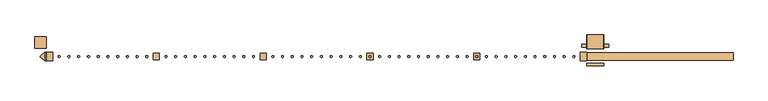
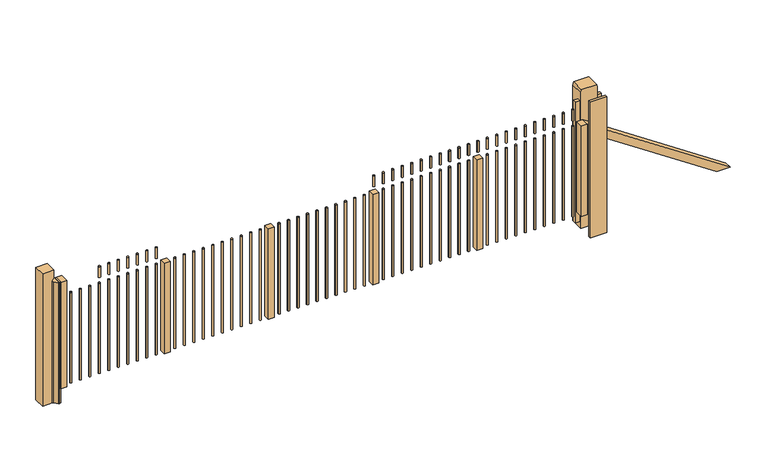
"""IFC4 building model written with IfcOpenShell, lengths in millimetres: door geometry, NLRS_90_DO_UN_schuifpoort met spijlen_gen_rsf : schuifpoort automatisch bxh 7000x1800-NP."""

import ifcopenshell
import ifcopenshell.guid

model = None  # the IFC model being written
_history = None  # IfcOwnerHistory: only IFC2X3 demands one
_inside = {}  # id of a spatial element -> (the spatial element, [elements in it])
_under = {}  # id of a project, library or spatial element -> (it, [spatial elements below it])
_declared = {}  # id of a project -> (the project, [libraries it declares])
_typed = {}  # id of a type object -> (the type object, [elements of that type])
_made_of = {}  # id of a material, layer set ... -> (it, [elements and type objects made of it])


def new_model(schema):
    """Start an empty IFC model of exactly this schema.

    Asked for "IFC4X3", IfcOpenShell would pick the latest addendum, in which some entities
    have other attributes; the version numbers below select the first issue.
    IFC2X3 requires an IfcOwnerHistory on every rooted entity: one is made here for all.
    """
    global model, _history
    if schema == "IFC4X3":
        model = ifcopenshell.file(schema_version=(4, 3, 0, 0))
    else:
        model = ifcopenshell.file(schema=schema)
    _inside.clear()
    _under.clear()
    _declared.clear()
    _typed.clear()
    _made_of.clear()
    _history = None
    if model.schema == "IFC2X3":
        org = make("IfcOrganization", Name="unknown")
        user = make(
            "IfcPersonAndOrganization",
            ThePerson=make("IfcPerson", FamilyName="unknown"),
            TheOrganization=org,
        )
        app = make(
            "IfcApplication",
            ApplicationDeveloper=org,
            Version="unknown",
            ApplicationFullName="unknown",
            ApplicationIdentifier="unknown",
        )
        _history = make(
            "IfcOwnerHistory",
            OwningUser=user,
            OwningApplication=app,
            ChangeAction="ADDED",
            CreationDate=0,
        )
    return model


def make(cls, **values):
    """One entity of the class cls with the attributes given. An attribute that is None is left unset."""
    return model.create_entity(
        cls, **{name: value for name, value in values.items() if value is not None}
    )


def rooted(cls, **values):
    """An entity with a GlobalId (a new one), such as an element, a storey or a relation."""
    return make(cls, GlobalId=ifcopenshell.guid.new(), OwnerHistory=_history, **values)


def si_unit(unit_type, name, prefix=None):
    """IfcSIUnit, for example si_unit("LENGTHUNIT", "METRE", prefix="MILLI")."""
    return make("IfcSIUnit", UnitType=unit_type, Prefix=prefix, Name=name)


def assignment(units):
    """IfcUnitAssignment: the units of a project."""
    return None if units is None else make("IfcUnitAssignment", Units=units)


def point(xyz):
    """IfcCartesianPoint."""
    return None if xyz is None else make("IfcCartesianPoint", Coordinates=xyz)


def direction(xyz):
    """IfcDirection."""
    return None if xyz is None else make("IfcDirection", DirectionRatios=xyz)


def frame(location, z_axis=None, x_axis=None):
    """IfcAxis2Placement3D, a coordinate frame: its origin and axes. An axis left out is left unset."""
    return make(
        "IfcAxis2Placement3D",
        Location=point(location),
        Axis=direction(z_axis),
        RefDirection=direction(x_axis),
    )


def frame_2d(location, x_axis=None):
    """IfcAxis2Placement2D, a coordinate frame in the plane: its origin and x axis."""
    return make(
        "IfcAxis2Placement2D", Location=point(location), RefDirection=direction(x_axis)
    )


def origin():
    """The frame at (0, 0, 0) with its axes left unset."""
    return frame((0.0, 0.0, 0.0))


def place(relative_to, where):
    """IfcLocalPlacement: puts the frame where relative to a parent placement (None: the world)."""
    return make(
        "IfcLocalPlacement", PlacementRelTo=relative_to, RelativePlacement=where
    )


def context(
    kind, dimensions, precision=None, world=None, true_north=None, identifier=None
):
    """IfcGeometricRepresentationContext, for example the 3D "Model" context."""
    return make(
        "IfcGeometricRepresentationContext",
        ContextIdentifier=identifier,
        ContextType=kind,
        CoordinateSpaceDimension=dimensions,
        Precision=precision,
        WorldCoordinateSystem=world,
        TrueNorth=true_north,
    )


def project(units=None, contexts=None):
    """IfcProject with its units and contexts."""
    return rooted(
        "IfcProject",
        Name="project",
        RepresentationContexts=contexts,
        UnitsInContext=assignment(units),
    )


def spatial(cls, under=None, at=None, **own):
    """A site, building, storey or space (cls), placed at a placement, below another one or the project."""
    s = rooted(cls, ObjectPlacement=at, **own)
    if under is not None:
        _under.setdefault(under.id(), (under, []))[1].append(s)
    return s


def polyline(points):
    """IfcPolyline through the points."""
    return make("IfcPolyline", Points=[point(p) for p in points])


def circle_curve(where, radius):
    """IfcCircle in the frame where."""
    return make("IfcCircle", Position=where, Radius=radius)


def trimmed(basis, trim1, trim2, sense, master):
    """IfcTrimmedCurve: the piece of a basis curve between two trims."""
    return make(
        "IfcTrimmedCurve",
        BasisCurve=basis,
        Trim1=trim1,
        Trim2=trim2,
        SenseAgreement=sense,
        MasterRepresentation=master,
    )


def segment(curve, same_sense, transition):
    """IfcCompositeCurveSegment."""
    return make(
        "IfcCompositeCurveSegment",
        Transition=transition,
        SameSense=same_sense,
        ParentCurve=curve,
    )


def composite_curve(segments, self_intersect=None):
    """IfcCompositeCurve: segments joined end to end."""
    return make("IfcCompositeCurve", Segments=segments, SelfIntersect=self_intersect)


def outline(outer, holes=None, kind="AREA"):
    """IfcArbitraryClosedProfileDef: a profile drawn as a closed curve; with holes, ...WithVoids."""
    if holes is None:
        return make("IfcArbitraryClosedProfileDef", ProfileType=kind, OuterCurve=outer)
    return make(
        "IfcArbitraryProfileDefWithVoids",
        ProfileType=kind,
        OuterCurve=outer,
        InnerCurves=holes,
    )


def extrude(swept, where, along, depth):
    """IfcExtrudedAreaSolid: the profile swept, set in the frame where, extruded along a direction by depth."""
    return make(
        "IfcExtrudedAreaSolid",
        SweptArea=swept,
        Position=where,
        ExtrudedDirection=direction(along),
        Depth=depth,
    )


def shape(context_of_items, identifier, shape_type, items):
    """IfcShapeRepresentation: the items that make up one representation, for example the "Body"."""
    return make(
        "IfcShapeRepresentation",
        ContextOfItems=context_of_items,
        RepresentationIdentifier=identifier,
        RepresentationType=shape_type,
        Items=items,
    )


def source(mapping_origin, context_of_items, identifier, shape_type, items):
    """IfcRepresentationMap: a shape defined once, which mapped items show again and again."""
    return make(
        "IfcRepresentationMap",
        MappingOrigin=mapping_origin,
        MappedRepresentation=shape(context_of_items, identifier, shape_type, items),
    )


def transform(
    local_origin,
    x_axis=None,
    y_axis=None,
    z_axis=None,
    scale=None,
    scale2=None,
    scale3=None,
    uniform=True,
):
    """IfcCartesianTransformationOperator3D, or its non-uniform kind. x_axis, y_axis, z_axis: its Axis1, 2, 3."""
    if uniform:
        return make(
            "IfcCartesianTransformationOperator3D",
            Axis1=direction(x_axis),
            Axis2=direction(y_axis),
            LocalOrigin=point(local_origin),
            Scale=scale,
            Axis3=direction(z_axis),
        )
    return make(
        "IfcCartesianTransformationOperator3DnonUniform",
        Axis1=direction(x_axis),
        Axis2=direction(y_axis),
        LocalOrigin=point(local_origin),
        Scale=scale,
        Axis3=direction(z_axis),
        Scale2=scale2,
        Scale3=scale3,
    )


def mapped(mapping_source, mapping_target):
    """IfcMappedItem: shows the shape of a source again, moved by a transform."""
    return make(
        "IfcMappedItem", MappingSource=mapping_source, MappingTarget=mapping_target
    )


def made_of(thing, what):
    """Note that an element or type object is made of a material, layer set ...; save() writes the relation."""
    if what is not None:
        _made_of.setdefault(what.id(), (what, []))[1].append(thing)
    return thing


def element(
    cls,
    number,
    at=None,
    inside=None,
    cuts=None,
    type_object=None,
    material=None,
    context=None,
    identifier="Body",
    shape_type=None,
    held_by="IfcProductDefinitionShape",
    body=None,
    shapes=None,
    **own,
):
    """One element of the class cls, such as IfcWall. Its Tag is "e" and its number.

    at: its placement. inside: the storey or other place that contains it. cuts: it is an
    opening in that element (IfcRelVoidsElement). A single representation is given by context,
    identifier, shape_type and body (its items); several are given by shapes. held_by: the class
    of the entity that holds the representations. save() writes the other relations.
    """
    e = rooted(cls, Tag="e%d" % number, ObjectPlacement=at, **own)
    if body is not None:
        shapes = [shape(context, identifier, shape_type, body)]
    if shapes is not None:
        e.Representation = make(held_by, Representations=shapes)
    if inside is not None:
        _inside.setdefault(inside.id(), (inside, []))[1].append(e)
    if cuts is not None:
        rooted(
            "IfcRelVoidsElement", RelatingBuildingElement=cuts, RelatedOpeningElement=e
        )
    if type_object is not None:
        _typed.setdefault(type_object.id(), (type_object, []))[1].append(e)
    return made_of(e, material)


def aggregate(whole, parts):
    """IfcRelAggregates: a whole, such as a stair, and the parts it consists of."""
    return rooted("IfcRelAggregates", RelatingObject=whole, RelatedObjects=parts)


def save(model, path):
    """Write the relations noted so far, then the file.

    IfcRelAggregates (storeys below a building ...), IfcRelContainedInSpatialStructure (elements
    in a storey), IfcRelDefinesByType, IfcRelAssociatesMaterial and IfcRelDeclares: one each for
    every whole, place, type object, material and project.
    """
    for whole, parts in _under.values():
        aggregate(whole, parts)
    for where, things in _inside.values():
        rooted(
            "IfcRelContainedInSpatialStructure",
            RelatedElements=things,
            RelatingStructure=where,
        )
    for kind, things in _typed.values():
        rooted("IfcRelDefinesByType", RelatedObjects=things, RelatingType=kind)
    for what, things in _made_of.values():
        rooted("IfcRelAssociatesMaterial", RelatedObjects=things, RelatingMaterial=what)
    for by, libraries in _declared.values():
        rooted("IfcRelDeclares", RelatingContext=by, RelatedDefinitions=libraries)
    model.write(path)


def door_7189267d(model_context):
    return source(origin(), model_context, "Body", "SweptSolid", [
        extrude(outline(composite_curve([segment(trimmed(circle_curve(frame_2d((3299.5, 0.0)), 12.5), [point((3312.0, 0.0))], [point((3287.0, 0.0))], False, "CARTESIAN"), True, "CONTINUOUS"), segment(trimmed(circle_curve(frame_2d((3299.5, 0.0)), 12.5), [point((3287.0, 0.0))], [point((3312.0, 0.0))], False, "CARTESIAN"), True, "CONTINUOUS")], self_intersect=False)), frame((0.0, 0.0, 300.0), z_axis=(0.0, 0.0, 1.0), x_axis=(1.0, 0.0, 0.0)), (0.0, 0.0, 1.0), 1270.0),
        extrude(outline(composite_curve([segment(trimmed(circle_curve(frame_2d((3173.5, 0.0)), 12.5), [point((3186.0, 0.0))], [point((3161.0, 0.0))], False, "CARTESIAN"), True, "CONTINUOUS"), segment(trimmed(circle_curve(frame_2d((3173.5, 0.0)), 12.5), [point((3161.0, 0.0))], [point((3186.0, 0.0))], False, "CARTESIAN"), True, "CONTINUOUS")], self_intersect=False)), frame((0.0, 0.0, 300.0), z_axis=(0.0, 0.0, 1.0), x_axis=(1.0, 0.0, 0.0)), (0.0, 0.0, 1.0), 1270.0),
        extrude(outline(composite_curve([segment(trimmed(circle_curve(frame_2d((3047.5, 0.0)), 12.5), [point((3060.0, 0.0))], [point((3035.0, 0.0))], False, "CARTESIAN"), True, "CONTINUOUS"), segment(trimmed(circle_curve(frame_2d((3047.5, 0.0)), 12.5), [point((3035.0, 0.0))], [point((3060.0, 0.0))], False, "CARTESIAN"), True, "CONTINUOUS")], self_intersect=False)), frame((0.0, 0.0, 300.0), z_axis=(0.0, 0.0, 1.0), x_axis=(1.0, 0.0, 0.0)), (0.0, 0.0, 1.0), 1270.0),
        extrude(outline(composite_curve([segment(trimmed(circle_curve(frame_2d((2921.5, 0.0)), 12.5), [point((2934.0, 0.0))], [point((2909.0, 0.0))], False, "CARTESIAN"), True, "CONTINUOUS"), segment(trimmed(circle_curve(frame_2d((2921.5, 0.0)), 12.5), [point((2909.0, 0.0))], [point((2934.0, 0.0))], False, "CARTESIAN"), True, "CONTINUOUS")], self_intersect=False)), frame((0.0, 0.0, 300.0), z_axis=(0.0, 0.0, 1.0), x_axis=(1.0, 0.0, 0.0)), (0.0, 0.0, 1.0), 1270.0),
        extrude(outline(composite_curve([segment(trimmed(circle_curve(frame_2d((2795.5, 0.0)), 12.5), [point((2808.0, 0.0))], [point((2783.0, 0.0))], False, "CARTESIAN"), True, "CONTINUOUS"), segment(trimmed(circle_curve(frame_2d((2795.5, 0.0)), 12.5), [point((2783.0, 0.0))], [point((2808.0, 0.0))], False, "CARTESIAN"), True, "CONTINUOUS")], self_intersect=False)), frame((0.0, 0.0, 300.0), z_axis=(0.0, 0.0, 1.0), x_axis=(1.0, 0.0, 0.0)), (0.0, 0.0, 1.0), 1270.0),
        extrude(outline(composite_curve([segment(trimmed(circle_curve(frame_2d((2669.5, 0.0)), 12.5), [point((2682.0, 0.0))], [point((2657.0, 0.0))], False, "CARTESIAN"), True, "CONTINUOUS"), segment(trimmed(circle_curve(frame_2d((2669.5, 0.0)), 12.5), [point((2657.0, 0.0))], [point((2682.0, 0.0))], False, "CARTESIAN"), True, "CONTINUOUS")], self_intersect=False)), frame((0.0, 0.0, 300.0), z_axis=(0.0, 0.0, 1.0), x_axis=(1.0, 0.0, 0.0)), (0.0, 0.0, 1.0), 1270.0),
        extrude(outline(composite_curve([segment(trimmed(circle_curve(frame_2d((2543.5, 0.0)), 12.5), [point((2556.0, 0.0))], [point((2531.0, 0.0))], False, "CARTESIAN"), True, "CONTINUOUS"), segment(trimmed(circle_curve(frame_2d((2543.5, 0.0)), 12.5), [point((2531.0, 0.0))], [point((2556.0, 0.0))], False, "CARTESIAN"), True, "CONTINUOUS")], self_intersect=False)), frame((0.0, 0.0, 300.0), z_axis=(0.0, 0.0, 1.0), x_axis=(1.0, 0.0, 0.0)), (0.0, 0.0, 1.0), 1270.0),
        extrude(outline(composite_curve([segment(trimmed(circle_curve(frame_2d((2417.5, 0.0)), 12.5), [point((2430.0, 0.0))], [point((2405.0, 0.0))], False, "CARTESIAN"), True, "CONTINUOUS"), segment(trimmed(circle_curve(frame_2d((2417.5, 0.0)), 12.5), [point((2405.0, 0.0))], [point((2430.0, 0.0))], False, "CARTESIAN"), True, "CONTINUOUS")], self_intersect=False)), frame((0.0, 0.0, 300.0), z_axis=(0.0, 0.0, 1.0), x_axis=(1.0, 0.0, 0.0)), (0.0, 0.0, 1.0), 1270.0),
        extrude(outline(composite_curve([segment(trimmed(circle_curve(frame_2d((2291.5, 0.0)), 12.5), [point((2304.0, 0.0))], [point((2279.0, 0.0))], False, "CARTESIAN"), True, "CONTINUOUS"), segment(trimmed(circle_curve(frame_2d((2291.5, 0.0)), 12.5), [point((2279.0, 0.0))], [point((2304.0, 0.0))], False, "CARTESIAN"), True, "CONTINUOUS")], self_intersect=False)), frame((0.0, 0.0, 300.0), z_axis=(0.0, 0.0, 1.0), x_axis=(1.0, 0.0, 0.0)), (0.0, 0.0, 1.0), 1270.0),
        extrude(outline(composite_curve([segment(trimmed(circle_curve(frame_2d((2165.5, 0.0)), 12.5), [point((2178.0, 0.0))], [point((2153.0, 0.0))], False, "CARTESIAN"), True, "CONTINUOUS"), segment(trimmed(circle_curve(frame_2d((2165.5, 0.0)), 12.5), [point((2153.0, 0.0))], [point((2178.0, 0.0))], False, "CARTESIAN"), True, "CONTINUOUS")], self_intersect=False)), frame((0.0, 0.0, 300.0), z_axis=(0.0, 0.0, 1.0), x_axis=(1.0, 0.0, 0.0)), (0.0, 0.0, 1.0), 1270.0),
        extrude(outline(composite_curve([segment(trimmed(circle_curve(frame_2d((1915.5, 0.0)), 12.5), [point((1928.0, 0.0))], [point((1903.0, 0.0))], False, "CARTESIAN"), True, "CONTINUOUS"), segment(trimmed(circle_curve(frame_2d((1915.5, 0.0)), 12.5), [point((1903.0, 0.0))], [point((1928.0, 0.0))], False, "CARTESIAN"), True, "CONTINUOUS")], self_intersect=False)), frame((0.0, 0.0, 300.0), z_axis=(0.0, 0.0, 1.0), x_axis=(1.0, 0.0, 0.0)), (0.0, 0.0, 1.0), 1270.0),
        extrude(outline(composite_curve([segment(trimmed(circle_curve(frame_2d((1789.5, 0.0)), 12.5), [point((1802.0, 0.0))], [point((1777.0, 0.0))], False, "CARTESIAN"), True, "CONTINUOUS"), segment(trimmed(circle_curve(frame_2d((1789.5, 0.0)), 12.5), [point((1777.0, 0.0))], [point((1802.0, 0.0))], False, "CARTESIAN"), True, "CONTINUOUS")], self_intersect=False)), frame((0.0, 0.0, 300.0), z_axis=(0.0, 0.0, 1.0), x_axis=(1.0, 0.0, 0.0)), (0.0, 0.0, 1.0), 1270.0),
        extrude(outline(composite_curve([segment(trimmed(circle_curve(frame_2d((1663.5, 0.0)), 12.5), [point((1676.0, 0.0))], [point((1651.0, 0.0))], False, "CARTESIAN"), True, "CONTINUOUS"), segment(trimmed(circle_curve(frame_2d((1663.5, 0.0)), 12.5), [point((1651.0, 0.0))], [point((1676.0, 0.0))], False, "CARTESIAN"), True, "CONTINUOUS")], self_intersect=False)), frame((0.0, 0.0, 300.0), z_axis=(0.0, 0.0, 1.0), x_axis=(1.0, 0.0, 0.0)), (0.0, 0.0, 1.0), 1270.0),
        extrude(outline(composite_curve([segment(trimmed(circle_curve(frame_2d((1537.5, 0.0)), 12.5), [point((1550.0, 0.0))], [point((1525.0, 0.0))], False, "CARTESIAN"), True, "CONTINUOUS"), segment(trimmed(circle_curve(frame_2d((1537.5, 0.0)), 12.5), [point((1525.0, 0.0))], [point((1550.0, 0.0))], False, "CARTESIAN"), True, "CONTINUOUS")], self_intersect=False)), frame((0.0, 0.0, 300.0), z_axis=(0.0, 0.0, 1.0), x_axis=(1.0, 0.0, 0.0)), (0.0, 0.0, 1.0), 1270.0),
        extrude(outline(composite_curve([segment(trimmed(circle_curve(frame_2d((1411.5, 0.0)), 12.5), [point((1424.0, 0.0))], [point((1399.0, 0.0))], False, "CARTESIAN"), True, "CONTINUOUS"), segment(trimmed(circle_curve(frame_2d((1411.5, 0.0)), 12.5), [point((1399.0, 0.0))], [point((1424.0, 0.0))], False, "CARTESIAN"), True, "CONTINUOUS")], self_intersect=False)), frame((0.0, 0.0, 300.0), z_axis=(0.0, 0.0, 1.0), x_axis=(1.0, 0.0, 0.0)), (0.0, 0.0, 1.0), 1270.0),
        extrude(outline(composite_curve([segment(trimmed(circle_curve(frame_2d((1285.5, 0.0)), 12.5), [point((1298.0, 0.0))], [point((1273.0, 0.0))], False, "CARTESIAN"), True, "CONTINUOUS"), segment(trimmed(circle_curve(frame_2d((1285.5, 0.0)), 12.5), [point((1273.0, 0.0))], [point((1298.0, 0.0))], False, "CARTESIAN"), True, "CONTINUOUS")], self_intersect=False)), frame((0.0, 0.0, 300.0), z_axis=(0.0, 0.0, 1.0), x_axis=(1.0, 0.0, 0.0)), (0.0, 0.0, 1.0), 1270.0),
        extrude(outline(composite_curve([segment(trimmed(circle_curve(frame_2d((1159.5, 0.0)), 12.5), [point((1172.0, 0.0))], [point((1147.0, 0.0))], False, "CARTESIAN"), True, "CONTINUOUS"), segment(trimmed(circle_curve(frame_2d((1159.5, 0.0)), 12.5), [point((1147.0, 0.0))], [point((1172.0, 0.0))], False, "CARTESIAN"), True, "CONTINUOUS")], self_intersect=False)), frame((0.0, 0.0, 300.0), z_axis=(0.0, 0.0, 1.0), x_axis=(1.0, 0.0, 0.0)), (0.0, 0.0, 1.0), 1270.0),
        extrude(outline(composite_curve([segment(trimmed(circle_curve(frame_2d((1033.5, 0.0)), 12.5), [point((1046.0, 0.0))], [point((1021.0, 0.0))], False, "CARTESIAN"), True, "CONTINUOUS"), segment(trimmed(circle_curve(frame_2d((1033.5, 0.0)), 12.5), [point((1021.0, 0.0))], [point((1046.0, 0.0))], False, "CARTESIAN"), True, "CONTINUOUS")], self_intersect=False)), frame((0.0, 0.0, 300.0), z_axis=(0.0, 0.0, 1.0), x_axis=(1.0, 0.0, 0.0)), (0.0, 0.0, 1.0), 1270.0),
        extrude(outline(composite_curve([segment(trimmed(circle_curve(frame_2d((907.5, 0.0)), 12.5), [point((920.0, 0.0))], [point((895.0, 0.0))], False, "CARTESIAN"), True, "CONTINUOUS"), segment(trimmed(circle_curve(frame_2d((907.5, 0.0)), 12.5), [point((895.0, 0.0))], [point((920.0, 0.0))], False, "CARTESIAN"), True, "CONTINUOUS")], self_intersect=False)), frame((0.0, 0.0, 300.0), z_axis=(0.0, 0.0, 1.0), x_axis=(1.0, 0.0, 0.0)), (0.0, 0.0, 1.0), 1270.0),
        extrude(outline(composite_curve([segment(trimmed(circle_curve(frame_2d((781.5, 0.0)), 12.5), [point((794.0, 0.0))], [point((769.0, 0.0))], False, "CARTESIAN"), True, "CONTINUOUS"), segment(trimmed(circle_curve(frame_2d((781.5, 0.0)), 12.5), [point((769.0, 0.0))], [point((794.0, 0.0))], False, "CARTESIAN"), True, "CONTINUOUS")], self_intersect=False)), frame((0.0, 0.0, 300.0), z_axis=(0.0, 0.0, 1.0), x_axis=(1.0, 0.0, 0.0)), (0.0, 0.0, 1.0), 1270.0),
        extrude(outline(polyline([(3465.0, 158.5), (3465.0, 118.5), (3400.0, 118.5), (3400.0, 158.5), (3465.0, 158.5)])), frame((0.0, 0.0, 100.0), z_axis=(0.0, 0.0, 1.0), x_axis=(1.0, 0.0, 0.0)), (0.0, 0.0, 1.0), 1700.0),
        extrude(outline(polyline([(3685.0, 158.5), (3750.0, 158.5), (3750.0, 118.5), (3685.0, 118.5), (3685.0, 158.5)])), frame((0.0, 0.0, 100.0), z_axis=(0.0, 0.0, 1.0), x_axis=(1.0, 0.0, 0.0)), (0.0, 0.0, 1.0), 1700.0),
        extrude(outline(polyline([(3685.0, -84.5), (3685.0, -119.5), (3465.0, -119.5), (3465.0, -84.5), (3685.0, -84.5)])), frame((0.0, 0.0, 12.0), z_axis=(0.0, 0.0, 1.0), x_axis=(1.0, 0.0, 0.0)), (0.0, 0.0, 1.0), 1906.0),
        extrude(outline(polyline([(1918.0, 3465.0), (12.0, 3465.0), (12.0, 3685.0), (1918.0, 3685.0), (1960.0, 3677.5), (1960.0, 3472.5), (1918.0, 3465.0)])), frame((0.0, 100.5, 0.0), z_axis=(0.0, 1.0, 0.0), x_axis=(0.0, 0.0, 1.0)), (0.0, 0.0, 1.0), 180.0),
        extrude(outline(polyline([(2000.5, 40.0), (2080.5, 40.0), (2080.5, -40.0), (2000.5, -40.0), (2000.5, 40.0)])), frame((0.0, 0.0, 300.0), z_axis=(0.0, 0.0, 1.0), x_axis=(1.0, 0.0, 0.0)), (0.0, 0.0, 1.0), 1270.0),
        extrude(outline(polyline([(616.5, 40.0), (696.5, 40.0), (696.5, -40.0), (616.5, -40.0), (616.5, 40.0)])), frame((0.0, 0.0, 300.0), z_axis=(0.0, 0.0, 1.0), x_axis=(1.0, 0.0, 0.0)), (0.0, 0.0, 1.0), 1270.0),
        extrude(outline(polyline([(-767.5, 40.0), (-687.5, 40.0), (-687.5, -40.0), (-767.5, -40.0), (-767.5, 40.0)])), frame((0.0, 0.0, 300.0), z_axis=(0.0, 0.0, 1.0), x_axis=(1.0, 0.0, 0.0)), (0.0, 0.0, 1.0), 1270.0),
        extrude(outline(polyline([(-2151.5, 40.0), (-2071.5, 40.0), (-2071.5, -40.0), (-2151.5, -40.0), (-2151.5, 40.0)])), frame((0.0, 0.0, 300.0), z_axis=(0.0, 0.0, 1.0), x_axis=(1.0, 0.0, 0.0)), (0.0, 0.0, 1.0), 1270.0),
        extrude(outline(composite_curve([segment(trimmed(circle_curve(frame_2d((531.5, 0.0)), 12.5), [point((544.0, 0.0))], [point((519.0, 0.0))], False, "CARTESIAN"), True, "CONTINUOUS"), segment(trimmed(circle_curve(frame_2d((531.5, 0.0)), 12.5), [point((519.0, 0.0))], [point((544.0, 0.0))], False, "CARTESIAN"), True, "CONTINUOUS")], self_intersect=False)), frame((0.0, 0.0, 300.0), z_axis=(0.0, 0.0, 1.0), x_axis=(1.0, 0.0, 0.0)), (0.0, 0.0, 1.0), 1270.0),
        extrude(outline(composite_curve([segment(trimmed(circle_curve(frame_2d((405.5, 0.0)), 12.5), [point((418.0, 0.0))], [point((393.0, 0.0))], False, "CARTESIAN"), True, "CONTINUOUS"), segment(trimmed(circle_curve(frame_2d((405.5, 0.0)), 12.5), [point((393.0, 0.0))], [point((418.0, 0.0))], False, "CARTESIAN"), True, "CONTINUOUS")], self_intersect=False)), frame((0.0, 0.0, 300.0), z_axis=(0.0, 0.0, 1.0), x_axis=(1.0, 0.0, 0.0)), (0.0, 0.0, 1.0), 1270.0),
        extrude(outline(composite_curve([segment(trimmed(circle_curve(frame_2d((279.5, 0.0)), 12.5), [point((292.0, 0.0))], [point((267.0, 0.0))], False, "CARTESIAN"), True, "CONTINUOUS"), segment(trimmed(circle_curve(frame_2d((279.5, 0.0)), 12.5), [point((267.0, 0.0))], [point((292.0, 0.0))], False, "CARTESIAN"), True, "CONTINUOUS")], self_intersect=False)), frame((0.0, 0.0, 300.0), z_axis=(0.0, 0.0, 1.0), x_axis=(1.0, 0.0, 0.0)), (0.0, 0.0, 1.0), 1270.0),
        extrude(outline(composite_curve([segment(trimmed(circle_curve(frame_2d((153.5, 0.0)), 12.5), [point((166.0, 0.0))], [point((141.0, 0.0))], False, "CARTESIAN"), True, "CONTINUOUS"), segment(trimmed(circle_curve(frame_2d((153.5, 0.0)), 12.5), [point((141.0, 0.0))], [point((166.0, 0.0))], False, "CARTESIAN"), True, "CONTINUOUS")], self_intersect=False)), frame((0.0, 0.0, 300.0), z_axis=(0.0, 0.0, 1.0), x_axis=(1.0, 0.0, 0.0)), (0.0, 0.0, 1.0), 1270.0),
        extrude(outline(composite_curve([segment(trimmed(circle_curve(frame_2d((27.5, 0.0)), 12.5), [point((40.0, 0.0))], [point((15.0, 0.0))], False, "CARTESIAN"), True, "CONTINUOUS"), segment(trimmed(circle_curve(frame_2d((27.5, 0.0)), 12.5), [point((15.0, 0.0))], [point((40.0, 0.0))], False, "CARTESIAN"), True, "CONTINUOUS")], self_intersect=False)), frame((0.0, 0.0, 300.0), z_axis=(0.0, 0.0, 1.0), x_axis=(1.0, 0.0, 0.0)), (0.0, 0.0, 1.0), 1270.0),
        extrude(outline(composite_curve([segment(trimmed(circle_curve(frame_2d((-98.5, 0.0)), 12.5), [point((-86.0, 0.0))], [point((-111.0, 0.0))], False, "CARTESIAN"), True, "CONTINUOUS"), segment(trimmed(circle_curve(frame_2d((-98.5, 0.0)), 12.5), [point((-111.0, 0.0))], [point((-86.0, 0.0))], False, "CARTESIAN"), True, "CONTINUOUS")], self_intersect=False)), frame((0.0, 0.0, 300.0), z_axis=(0.0, 0.0, 1.0), x_axis=(1.0, 0.0, 0.0)), (0.0, 0.0, 1.0), 1270.0),
        extrude(outline(composite_curve([segment(trimmed(circle_curve(frame_2d((-224.5, 0.0)), 12.5), [point((-212.0, 0.0))], [point((-237.0, 0.0))], False, "CARTESIAN"), True, "CONTINUOUS"), segment(trimmed(circle_curve(frame_2d((-224.5, 0.0)), 12.5), [point((-237.0, 0.0))], [point((-212.0, 0.0))], False, "CARTESIAN"), True, "CONTINUOUS")], self_intersect=False)), frame((0.0, 0.0, 300.0), z_axis=(0.0, 0.0, 1.0), x_axis=(1.0, 0.0, 0.0)), (0.0, 0.0, 1.0), 1270.0),
        extrude(outline(composite_curve([segment(trimmed(circle_curve(frame_2d((-350.5, 0.0)), 12.5), [point((-338.0, 0.0))], [point((-363.0, 0.0))], False, "CARTESIAN"), True, "CONTINUOUS"), segment(trimmed(circle_curve(frame_2d((-350.5, 0.0)), 12.5), [point((-363.0, 0.0))], [point((-338.0, 0.0))], False, "CARTESIAN"), True, "CONTINUOUS")], self_intersect=False)), frame((0.0, 0.0, 300.0), z_axis=(0.0, 0.0, 1.0), x_axis=(1.0, 0.0, 0.0)), (0.0, 0.0, 1.0), 1270.0),
        extrude(outline(composite_curve([segment(trimmed(circle_curve(frame_2d((-476.5, 0.0)), 12.5), [point((-464.0, 0.0))], [point((-489.0, 0.0))], False, "CARTESIAN"), True, "CONTINUOUS"), segment(trimmed(circle_curve(frame_2d((-476.5, 0.0)), 12.5), [point((-489.0, 0.0))], [point((-464.0, 0.0))], False, "CARTESIAN"), True, "CONTINUOUS")], self_intersect=False)), frame((0.0, 0.0, 300.0), z_axis=(0.0, 0.0, 1.0), x_axis=(1.0, 0.0, 0.0)), (0.0, 0.0, 1.0), 1270.0),
        extrude(outline(composite_curve([segment(trimmed(circle_curve(frame_2d((-602.5, 0.0)), 12.5), [point((-590.0, 0.0))], [point((-615.0, 0.0))], False, "CARTESIAN"), True, "CONTINUOUS"), segment(trimmed(circle_curve(frame_2d((-602.5, 0.0)), 12.5), [point((-615.0, 0.0))], [point((-590.0, 0.0))], False, "CARTESIAN"), True, "CONTINUOUS")], self_intersect=False)), frame((0.0, 0.0, 300.0), z_axis=(0.0, 0.0, 1.0), x_axis=(1.0, 0.0, 0.0)), (0.0, 0.0, 1.0), 1270.0),
        extrude(outline(polyline([(300.0, 5362.0), (1570.0, 3464.5), (1449.6685917, 3464.5), (300.0, 5182.2135061), (300.0, 5362.0)])), frame((0.0, -50.0, 0.0), z_axis=(0.0, 1.0, 0.0), x_axis=(0.0, 0.0, 1.0)), (0.0, 0.0, 1.0), 100.0),
        extrude(outline(composite_curve([segment(trimmed(circle_curve(frame_2d((-852.5, 0.0)), 12.5), [point((-840.0, 0.0))], [point((-865.0, 0.0))], False, "CARTESIAN"), True, "CONTINUOUS"), segment(trimmed(circle_curve(frame_2d((-852.5, 0.0)), 12.5), [point((-865.0, 0.0))], [point((-840.0, 0.0))], False, "CARTESIAN"), True, "CONTINUOUS")], self_intersect=False)), frame((0.0, 0.0, 300.0), z_axis=(0.0, 0.0, 1.0), x_axis=(1.0, 0.0, 0.0)), (0.0, 0.0, 1.0), 1270.0),
        extrude(outline(composite_curve([segment(trimmed(circle_curve(frame_2d((-978.5, 0.0)), 12.5), [point((-966.0, 0.0))], [point((-991.0, 0.0))], False, "CARTESIAN"), True, "CONTINUOUS"), segment(trimmed(circle_curve(frame_2d((-978.5, 0.0)), 12.5), [point((-991.0, 0.0))], [point((-966.0, 0.0))], False, "CARTESIAN"), True, "CONTINUOUS")], self_intersect=False)), frame((0.0, 0.0, 300.0), z_axis=(0.0, 0.0, 1.0), x_axis=(1.0, 0.0, 0.0)), (0.0, 0.0, 1.0), 1270.0),
        extrude(outline(composite_curve([segment(trimmed(circle_curve(frame_2d((-1104.5, 0.0)), 12.5), [point((-1092.0, 0.0))], [point((-1117.0, 0.0))], False, "CARTESIAN"), True, "CONTINUOUS"), segment(trimmed(circle_curve(frame_2d((-1104.5, 0.0)), 12.5), [point((-1117.0, 0.0))], [point((-1092.0, 0.0))], False, "CARTESIAN"), True, "CONTINUOUS")], self_intersect=False)), frame((0.0, 0.0, 300.0), z_axis=(0.0, 0.0, 1.0), x_axis=(1.0, 0.0, 0.0)), (0.0, 0.0, 1.0), 1270.0),
        extrude(outline(composite_curve([segment(trimmed(circle_curve(frame_2d((-1230.5, 0.0)), 12.5), [point((-1218.0, 0.0))], [point((-1243.0, 0.0))], False, "CARTESIAN"), True, "CONTINUOUS"), segment(trimmed(circle_curve(frame_2d((-1230.5, 0.0)), 12.5), [point((-1243.0, 0.0))], [point((-1218.0, 0.0))], False, "CARTESIAN"), True, "CONTINUOUS")], self_intersect=False)), frame((0.0, 0.0, 300.0), z_axis=(0.0, 0.0, 1.0), x_axis=(1.0, 0.0, 0.0)), (0.0, 0.0, 1.0), 1270.0),
        extrude(outline(composite_curve([segment(trimmed(circle_curve(frame_2d((-1356.5, 0.0)), 12.5), [point((-1344.0, 0.0))], [point((-1369.0, 0.0))], False, "CARTESIAN"), True, "CONTINUOUS"), segment(trimmed(circle_curve(frame_2d((-1356.5, 0.0)), 12.5), [point((-1369.0, 0.0))], [point((-1344.0, 0.0))], False, "CARTESIAN"), True, "CONTINUOUS")], self_intersect=False)), frame((0.0, 0.0, 300.0), z_axis=(0.0, 0.0, 1.0), x_axis=(1.0, 0.0, 0.0)), (0.0, 0.0, 1.0), 1270.0),
        extrude(outline(composite_curve([segment(trimmed(circle_curve(frame_2d((-1482.5, 0.0)), 12.5), [point((-1470.0, 0.0))], [point((-1495.0, 0.0))], False, "CARTESIAN"), True, "CONTINUOUS"), segment(trimmed(circle_curve(frame_2d((-1482.5, 0.0)), 12.5), [point((-1495.0, 0.0))], [point((-1470.0, 0.0))], False, "CARTESIAN"), True, "CONTINUOUS")], self_intersect=False)), frame((0.0, 0.0, 300.0), z_axis=(0.0, 0.0, 1.0), x_axis=(1.0, 0.0, 0.0)), (0.0, 0.0, 1.0), 1270.0),
        extrude(outline(composite_curve([segment(trimmed(circle_curve(frame_2d((-1608.5, 0.0)), 12.5), [point((-1596.0, 0.0))], [point((-1621.0, 0.0))], False, "CARTESIAN"), True, "CONTINUOUS"), segment(trimmed(circle_curve(frame_2d((-1608.5, 0.0)), 12.5), [point((-1621.0, 0.0))], [point((-1596.0, 0.0))], False, "CARTESIAN"), True, "CONTINUOUS")], self_intersect=False)), frame((0.0, 0.0, 300.0), z_axis=(0.0, 0.0, 1.0), x_axis=(1.0, 0.0, 0.0)), (0.0, 0.0, 1.0), 1270.0),
        extrude(outline(composite_curve([segment(trimmed(circle_curve(frame_2d((-1734.5, 0.0)), 12.5), [point((-1722.0, 0.0))], [point((-1747.0, 0.0))], False, "CARTESIAN"), True, "CONTINUOUS"), segment(trimmed(circle_curve(frame_2d((-1734.5, 0.0)), 12.5), [point((-1747.0, 0.0))], [point((-1722.0, 0.0))], False, "CARTESIAN"), True, "CONTINUOUS")], self_intersect=False)), frame((0.0, 0.0, 300.0), z_axis=(0.0, 0.0, 1.0), x_axis=(1.0, 0.0, 0.0)), (0.0, 0.0, 1.0), 1270.0),
        extrude(outline(composite_curve([segment(trimmed(circle_curve(frame_2d((-1860.5, 0.0)), 12.5), [point((-1848.0, 0.0))], [point((-1873.0, 0.0))], False, "CARTESIAN"), True, "CONTINUOUS"), segment(trimmed(circle_curve(frame_2d((-1860.5, 0.0)), 12.5), [point((-1873.0, 0.0))], [point((-1848.0, 0.0))], False, "CARTESIAN"), True, "CONTINUOUS")], self_intersect=False)), frame((0.0, 0.0, 300.0), z_axis=(0.0, 0.0, 1.0), x_axis=(1.0, 0.0, 0.0)), (0.0, 0.0, 1.0), 1270.0),
        extrude(outline(composite_curve([segment(trimmed(circle_curve(frame_2d((-1986.5, 0.0)), 12.5), [point((-1974.0, 0.0))], [point((-1999.0, 0.0))], False, "CARTESIAN"), True, "CONTINUOUS"), segment(trimmed(circle_curve(frame_2d((-1986.5, 0.0)), 12.5), [point((-1999.0, 0.0))], [point((-1974.0, 0.0))], False, "CARTESIAN"), True, "CONTINUOUS")], self_intersect=False)), frame((0.0, 0.0, 300.0), z_axis=(0.0, 0.0, 1.0), x_axis=(1.0, 0.0, 0.0)), (0.0, 0.0, 1.0), 1270.0),
        extrude(outline(composite_curve([segment(trimmed(circle_curve(frame_2d((-2236.0, 0.0)), 12.5), [point((-2223.5, 0.0))], [point((-2248.5, 0.0))], False, "CARTESIAN"), True, "CONTINUOUS"), segment(trimmed(circle_curve(frame_2d((-2236.0, 0.0)), 12.5), [point((-2248.5, 0.0))], [point((-2223.5, 0.0))], False, "CARTESIAN"), True, "CONTINUOUS")], self_intersect=False)), frame((0.0, 0.0, 300.0), z_axis=(0.0, 0.0, 1.0), x_axis=(1.0, 0.0, 0.0)), (0.0, 0.0, 1.0), 1270.0),
        extrude(outline(composite_curve([segment(trimmed(circle_curve(frame_2d((-2362.0, 0.0)), 12.5), [point((-2349.5, 0.0))], [point((-2374.5, 0.0))], False, "CARTESIAN"), True, "CONTINUOUS"), segment(trimmed(circle_curve(frame_2d((-2362.0, 0.0)), 12.5), [point((-2374.5, 0.0))], [point((-2349.5, 0.0))], False, "CARTESIAN"), True, "CONTINUOUS")], self_intersect=False)), frame((0.0, 0.0, 300.0), z_axis=(0.0, 0.0, 1.0), x_axis=(1.0, 0.0, 0.0)), (0.0, 0.0, 1.0), 1270.0),
        extrude(outline(composite_curve([segment(trimmed(circle_curve(frame_2d((-2488.0, 0.0)), 12.5), [point((-2475.5, 0.0))], [point((-2500.5, 0.0))], False, "CARTESIAN"), True, "CONTINUOUS"), segment(trimmed(circle_curve(frame_2d((-2488.0, 0.0)), 12.5), [point((-2500.5, 0.0))], [point((-2475.5, 0.0))], False, "CARTESIAN"), True, "CONTINUOUS")], self_intersect=False)), frame((0.0, 0.0, 300.0), z_axis=(0.0, 0.0, 1.0), x_axis=(1.0, 0.0, 0.0)), (0.0, 0.0, 1.0), 1270.0),
        extrude(outline(composite_curve([segment(trimmed(circle_curve(frame_2d((-2614.0, 0.0)), 12.5), [point((-2601.5, 0.0))], [point((-2626.5, 0.0))], False, "CARTESIAN"), True, "CONTINUOUS"), segment(trimmed(circle_curve(frame_2d((-2614.0, 0.0)), 12.5), [point((-2626.5, 0.0))], [point((-2601.5, 0.0))], False, "CARTESIAN"), True, "CONTINUOUS")], self_intersect=False)), frame((0.0, 0.0, 300.0), z_axis=(0.0, 0.0, 1.0), x_axis=(1.0, 0.0, 0.0)), (0.0, 0.0, 1.0), 1270.0),
        extrude(outline(composite_curve([segment(trimmed(circle_curve(frame_2d((-2740.0, 0.0)), 12.5), [point((-2727.5, 0.0))], [point((-2752.5, 0.0))], False, "CARTESIAN"), True, "CONTINUOUS"), segment(trimmed(circle_curve(frame_2d((-2740.0, 0.0)), 12.5), [point((-2752.5, 0.0))], [point((-2727.5, 0.0))], False, "CARTESIAN"), True, "CONTINUOUS")], self_intersect=False)), frame((0.0, 0.0, 300.0), z_axis=(0.0, 0.0, 1.0), x_axis=(1.0, 0.0, 0.0)), (0.0, 0.0, 1.0), 1270.0),
        extrude(outline(composite_curve([segment(trimmed(circle_curve(frame_2d((-2866.0, 0.0)), 12.5), [point((-2853.5, 0.0))], [point((-2878.5, 0.0))], False, "CARTESIAN"), True, "CONTINUOUS"), segment(trimmed(circle_curve(frame_2d((-2866.0, 0.0)), 12.5), [point((-2878.5, 0.0))], [point((-2853.5, 0.0))], False, "CARTESIAN"), True, "CONTINUOUS")], self_intersect=False)), frame((0.0, 0.0, 300.0), z_axis=(0.0, 0.0, 1.0), x_axis=(1.0, 0.0, 0.0)), (0.0, 0.0, 1.0), 1270.0),
        extrude(outline(composite_curve([segment(trimmed(circle_curve(frame_2d((-2992.0, 0.0)), 12.5), [point((-2979.5, 0.0))], [point((-3004.5, 0.0))], False, "CARTESIAN"), True, "CONTINUOUS"), segment(trimmed(circle_curve(frame_2d((-2992.0, 0.0)), 12.5), [point((-3004.5, 0.0))], [point((-2979.5, 0.0))], False, "CARTESIAN"), True, "CONTINUOUS")], self_intersect=False)), frame((0.0, 0.0, 300.0), z_axis=(0.0, 0.0, 1.0), x_axis=(1.0, 0.0, 0.0)), (0.0, 0.0, 1.0), 1270.0),
        extrude(outline(composite_curve([segment(trimmed(circle_curve(frame_2d((-3118.0, 0.0)), 12.5), [point((-3105.5, 0.0))], [point((-3130.5, 0.0))], False, "CARTESIAN"), True, "CONTINUOUS"), segment(trimmed(circle_curve(frame_2d((-3118.0, 0.0)), 12.5), [point((-3130.5, 0.0))], [point((-3105.5, 0.0))], False, "CARTESIAN"), True, "CONTINUOUS")], self_intersect=False)), frame((0.0, 0.0, 300.0), z_axis=(0.0, 0.0, 1.0), x_axis=(1.0, 0.0, 0.0)), (0.0, 0.0, 1.0), 1270.0),
        extrude(outline(composite_curve([segment(trimmed(circle_curve(frame_2d((-3244.0, 0.0)), 12.5), [point((-3231.5, 0.0))], [point((-3256.5, 0.0))], False, "CARTESIAN"), True, "CONTINUOUS"), segment(trimmed(circle_curve(frame_2d((-3244.0, 0.0)), 12.5), [point((-3256.5, 0.0))], [point((-3231.5, 0.0))], False, "CARTESIAN"), True, "CONTINUOUS")], self_intersect=False)), frame((0.0, 0.0, 300.0), z_axis=(0.0, 0.0, 1.0), x_axis=(1.0, 0.0, 0.0)), (0.0, 0.0, 1.0), 1270.0),
        extrude(outline(composite_curve([segment(trimmed(circle_curve(frame_2d((-3370.0, 0.0)), 12.5), [point((-3357.5, 0.0))], [point((-3382.5, 0.0))], False, "CARTESIAN"), True, "CONTINUOUS"), segment(trimmed(circle_curve(frame_2d((-3370.0, 0.0)), 12.5), [point((-3382.5, 0.0))], [point((-3357.5, 0.0))], False, "CARTESIAN"), True, "CONTINUOUS")], self_intersect=False)), frame((0.0, 0.0, 300.0), z_axis=(0.0, 0.0, 1.0), x_axis=(1.0, 0.0, 0.0)), (0.0, 0.0, 1.0), 1270.0),
        extrude(outline(composite_curve([segment(polyline([(-3558.78125, -54.1621094), (-3609.625, -11.4902343)]), True, "CONTINUOUS"), segment(trimmed(circle_curve(frame_2d((-3600.0040885, 0.0)), 14.9862412), [point((-3609.625, -11.4902343))], [point((-3609.625, 11.4902343))], False, "CARTESIAN"), True, "CONTINUOUS"), segment(polyline([(-3609.625, 11.4902343), (-3558.765625, 54.1777344)]), True, "CONTINUOUS"), segment(trimmed(circle_curve(frame_2d((-3557.4950392, 52.6395691)), 1.9950791), [point((-3558.765625, 54.1777344))], [point((-3555.53125, 52.2876138))], False, "CARTESIAN"), True, "CONTINUOUS"), segment(polyline([(-3555.53125, 52.2876138), (-3555.53125, -52.8919162)]), True, "CONTINUOUS"), segment(trimmed(circle_curve(frame_2d((-3557.5075149, -52.6282432)), 1.9937769), [point((-3555.53125, -52.8919162))], [point((-3558.78125, -54.1621094))], False, "CARTESIAN"), True, "CONTINUOUS")], self_intersect=False)), frame((0.0, 0.0, 100.0), z_axis=(0.0, 0.0, 1.0), x_axis=(1.0, 0.0, 0.0)), (0.0, 0.0, 1.0), 1700.0),
        extrude(outline(polyline([(-3535.5, 52.8125), (-3535.5, -52.8125), (-3555.53125, -52.8125), (-3555.53125, 52.8125), (-3535.5, 52.8125)])), frame((0.0, 0.0, 100.0), z_axis=(0.0, 0.0, 1.0), x_axis=(1.0, 0.0, 0.0)), (0.0, 0.0, 1.0), 1700.0),
        extrude(outline(polyline([(-3535.0, 255.5), (-3535.0, 105.5), (-3685.0, 105.5), (-3685.0, 255.5), (-3535.0, 255.5)])), frame((0.0, 0.0, 12.0), z_axis=(0.0, 0.0, 1.0), x_axis=(1.0, 0.0, 0.0)), (0.0, 0.0, 1.0), 1861.0),
        extrude(outline(polyline([(3464.5, 55.0), (3464.5, -55.0), (3384.5, -55.0), (3384.5, 55.0), (3464.5, 55.0)])), frame((0.0, 0.0, 300.0), z_axis=(0.0, 0.0, 1.0), x_axis=(1.0, 0.0, 0.0)), (0.0, 0.0, 1.0), 1270.0),
        extrude(outline(polyline([(-3455.5, 55.0), (-3455.5, -55.0), (-3535.5, -55.0), (-3535.5, 55.0), (-3455.5, 55.0)])), frame((0.0, 0.0, 300.0), z_axis=(0.0, 0.0, 1.0), x_axis=(1.0, 0.0, 0.0)), (0.0, 0.0, 1.0), 1500.0),
        extrude(outline(composite_curve([segment(trimmed(circle_curve(frame_2d((3299.5, 0.0)), 12.5), [point((3312.0, 0.0))], [point((3287.0, 0.0))], False, "CARTESIAN"), True, "CONTINUOUS"), segment(trimmed(circle_curve(frame_2d((3299.5, 0.0)), 12.5), [point((3287.0, 0.0))], [point((3312.0, 0.0))], False, "CARTESIAN"), True, "CONTINUOUS")], self_intersect=False)), frame((0.0, 0.0, 1650.0), z_axis=(0.0, 0.0, 1.0), x_axis=(1.0, 0.0, 0.0)), (0.0, 0.0, 1.0), 150.0),
        extrude(outline(composite_curve([segment(trimmed(circle_curve(frame_2d((3173.5, 0.0)), 12.5), [point((3186.0, 0.0))], [point((3161.0, 0.0))], False, "CARTESIAN"), True, "CONTINUOUS"), segment(trimmed(circle_curve(frame_2d((3173.5, 0.0)), 12.5), [point((3161.0, 0.0))], [point((3186.0, 0.0))], False, "CARTESIAN"), True, "CONTINUOUS")], self_intersect=False)), frame((0.0, 0.0, 1650.0), z_axis=(0.0, 0.0, 1.0), x_axis=(1.0, 0.0, 0.0)), (0.0, 0.0, 1.0), 150.0),
        extrude(outline(composite_curve([segment(trimmed(circle_curve(frame_2d((3047.5, 0.0)), 12.5), [point((3060.0, 0.0))], [point((3035.0, 0.0))], False, "CARTESIAN"), True, "CONTINUOUS"), segment(trimmed(circle_curve(frame_2d((3047.5, 0.0)), 12.5), [point((3035.0, 0.0))], [point((3060.0, 0.0))], False, "CARTESIAN"), True, "CONTINUOUS")], self_intersect=False)), frame((0.0, 0.0, 1650.0), z_axis=(0.0, 0.0, 1.0), x_axis=(1.0, 0.0, 0.0)), (0.0, 0.0, 1.0), 150.0),
        extrude(outline(composite_curve([segment(trimmed(circle_curve(frame_2d((2921.5, 0.0)), 12.5), [point((2934.0, 0.0))], [point((2909.0, 0.0))], False, "CARTESIAN"), True, "CONTINUOUS"), segment(trimmed(circle_curve(frame_2d((2921.5, 0.0)), 12.5), [point((2909.0, 0.0))], [point((2934.0, 0.0))], False, "CARTESIAN"), True, "CONTINUOUS")], self_intersect=False)), frame((0.0, 0.0, 1650.0), z_axis=(0.0, 0.0, 1.0), x_axis=(1.0, 0.0, 0.0)), (0.0, 0.0, 1.0), 150.0),
        extrude(outline(composite_curve([segment(trimmed(circle_curve(frame_2d((2795.5, 0.0)), 12.5), [point((2808.0, 0.0))], [point((2783.0, 0.0))], False, "CARTESIAN"), True, "CONTINUOUS"), segment(trimmed(circle_curve(frame_2d((2795.5, 0.0)), 12.5), [point((2783.0, 0.0))], [point((2808.0, 0.0))], False, "CARTESIAN"), True, "CONTINUOUS")], self_intersect=False)), frame((0.0, 0.0, 1650.0), z_axis=(0.0, 0.0, 1.0), x_axis=(1.0, 0.0, 0.0)), (0.0, 0.0, 1.0), 150.0),
        extrude(outline(composite_curve([segment(trimmed(circle_curve(frame_2d((2669.5, 0.0)), 12.5), [point((2682.0, 0.0))], [point((2657.0, 0.0))], False, "CARTESIAN"), True, "CONTINUOUS"), segment(trimmed(circle_curve(frame_2d((2669.5, 0.0)), 12.5), [point((2657.0, 0.0))], [point((2682.0, 0.0))], False, "CARTESIAN"), True, "CONTINUOUS")], self_intersect=False)), frame((0.0, 0.0, 1650.0), z_axis=(0.0, 0.0, 1.0), x_axis=(1.0, 0.0, 0.0)), (0.0, 0.0, 1.0), 150.0),
        extrude(outline(composite_curve([segment(trimmed(circle_curve(frame_2d((2543.5, 0.0)), 12.5), [point((2556.0, 0.0))], [point((2531.0, 0.0))], False, "CARTESIAN"), True, "CONTINUOUS"), segment(trimmed(circle_curve(frame_2d((2543.5, 0.0)), 12.5), [point((2531.0, 0.0))], [point((2556.0, 0.0))], False, "CARTESIAN"), True, "CONTINUOUS")], self_intersect=False)), frame((0.0, 0.0, 1650.0), z_axis=(0.0, 0.0, 1.0), x_axis=(1.0, 0.0, 0.0)), (0.0, 0.0, 1.0), 150.0),
        extrude(outline(composite_curve([segment(trimmed(circle_curve(frame_2d((2417.5, 0.0)), 12.5), [point((2430.0, 0.0))], [point((2405.0, 0.0))], False, "CARTESIAN"), True, "CONTINUOUS"), segment(trimmed(circle_curve(frame_2d((2417.5, 0.0)), 12.5), [point((2405.0, 0.0))], [point((2430.0, 0.0))], False, "CARTESIAN"), True, "CONTINUOUS")], self_intersect=False)), frame((0.0, 0.0, 1650.0), z_axis=(0.0, 0.0, 1.0), x_axis=(1.0, 0.0, 0.0)), (0.0, 0.0, 1.0), 150.0),
        extrude(outline(composite_curve([segment(trimmed(circle_curve(frame_2d((2291.5, 0.0)), 12.5), [point((2304.0, 0.0))], [point((2279.0, 0.0))], False, "CARTESIAN"), True, "CONTINUOUS"), segment(trimmed(circle_curve(frame_2d((2291.5, 0.0)), 12.5), [point((2279.0, 0.0))], [point((2304.0, 0.0))], False, "CARTESIAN"), True, "CONTINUOUS")], self_intersect=False)), frame((0.0, 0.0, 1650.0), z_axis=(0.0, 0.0, 1.0), x_axis=(1.0, 0.0, 0.0)), (0.0, 0.0, 1.0), 150.0),
        extrude(outline(composite_curve([segment(trimmed(circle_curve(frame_2d((2165.5, 0.0)), 12.5), [point((2178.0, 0.0))], [point((2153.0, 0.0))], False, "CARTESIAN"), True, "CONTINUOUS"), segment(trimmed(circle_curve(frame_2d((2165.5, 0.0)), 12.5), [point((2153.0, 0.0))], [point((2178.0, 0.0))], False, "CARTESIAN"), True, "CONTINUOUS")], self_intersect=False)), frame((0.0, 0.0, 1650.0), z_axis=(0.0, 0.0, 1.0), x_axis=(1.0, 0.0, 0.0)), (0.0, 0.0, 1.0), 150.0),
        extrude(outline(composite_curve([segment(trimmed(circle_curve(frame_2d((2040.5, 0.0)), 12.5), [point((2053.0, 0.0))], [point((2028.0, 0.0))], False, "CARTESIAN"), True, "CONTINUOUS"), segment(trimmed(circle_curve(frame_2d((2040.5, 0.0)), 12.5), [point((2028.0, 0.0))], [point((2053.0, 0.0))], False, "CARTESIAN"), True, "CONTINUOUS")], self_intersect=False)), frame((0.0, 0.0, 1650.0), z_axis=(0.0, 0.0, 1.0), x_axis=(1.0, 0.0, 0.0)), (0.0, 0.0, 1.0), 150.0),
        extrude(outline(composite_curve([segment(trimmed(circle_curve(frame_2d((656.5, 0.0)), 12.5), [point((669.0, 0.0))], [point((644.0, 0.0))], False, "CARTESIAN"), True, "CONTINUOUS"), segment(trimmed(circle_curve(frame_2d((656.5, 0.0)), 12.5), [point((644.0, 0.0))], [point((669.0, 0.0))], False, "CARTESIAN"), True, "CONTINUOUS")], self_intersect=False)), frame((0.0, 0.0, 1650.0), z_axis=(0.0, 0.0, 1.0), x_axis=(1.0, 0.0, 0.0)), (0.0, 0.0, 1.0), 150.0),
        extrude(outline(composite_curve([segment(trimmed(circle_curve(frame_2d((1915.5, 0.0)), 12.5), [point((1928.0, 0.0))], [point((1903.0, 0.0))], False, "CARTESIAN"), True, "CONTINUOUS"), segment(trimmed(circle_curve(frame_2d((1915.5, 0.0)), 12.5), [point((1903.0, 0.0))], [point((1928.0, 0.0))], False, "CARTESIAN"), True, "CONTINUOUS")], self_intersect=False)), frame((0.0, 0.0, 1650.0), z_axis=(0.0, 0.0, 1.0), x_axis=(1.0, 0.0, 0.0)), (0.0, 0.0, 1.0), 150.0),
        extrude(outline(composite_curve([segment(trimmed(circle_curve(frame_2d((1789.5, 0.0)), 12.5), [point((1802.0, 0.0))], [point((1777.0, 0.0))], False, "CARTESIAN"), True, "CONTINUOUS"), segment(trimmed(circle_curve(frame_2d((1789.5, 0.0)), 12.5), [point((1777.0, 0.0))], [point((1802.0, 0.0))], False, "CARTESIAN"), True, "CONTINUOUS")], self_intersect=False)), frame((0.0, 0.0, 1650.0), z_axis=(0.0, 0.0, 1.0), x_axis=(1.0, 0.0, 0.0)), (0.0, 0.0, 1.0), 150.0),
        extrude(outline(composite_curve([segment(trimmed(circle_curve(frame_2d((1663.5, 0.0)), 12.5), [point((1676.0, 0.0))], [point((1651.0, 0.0))], False, "CARTESIAN"), True, "CONTINUOUS"), segment(trimmed(circle_curve(frame_2d((1663.5, 0.0)), 12.5), [point((1651.0, 0.0))], [point((1676.0, 0.0))], False, "CARTESIAN"), True, "CONTINUOUS")], self_intersect=False)), frame((0.0, 0.0, 1650.0), z_axis=(0.0, 0.0, 1.0), x_axis=(1.0, 0.0, 0.0)), (0.0, 0.0, 1.0), 150.0),
        extrude(outline(composite_curve([segment(trimmed(circle_curve(frame_2d((1537.5, 0.0)), 12.5), [point((1550.0, 0.0))], [point((1525.0, 0.0))], False, "CARTESIAN"), True, "CONTINUOUS"), segment(trimmed(circle_curve(frame_2d((1537.5, 0.0)), 12.5), [point((1525.0, 0.0))], [point((1550.0, 0.0))], False, "CARTESIAN"), True, "CONTINUOUS")], self_intersect=False)), frame((0.0, 0.0, 1650.0), z_axis=(0.0, 0.0, 1.0), x_axis=(1.0, 0.0, 0.0)), (0.0, 0.0, 1.0), 150.0),
        extrude(outline(composite_curve([segment(trimmed(circle_curve(frame_2d((1411.5, 0.0)), 12.5), [point((1424.0, 0.0))], [point((1399.0, 0.0))], False, "CARTESIAN"), True, "CONTINUOUS"), segment(trimmed(circle_curve(frame_2d((1411.5, 0.0)), 12.5), [point((1399.0, 0.0))], [point((1424.0, 0.0))], False, "CARTESIAN"), True, "CONTINUOUS")], self_intersect=False)), frame((0.0, 0.0, 1650.0), z_axis=(0.0, 0.0, 1.0), x_axis=(1.0, 0.0, 0.0)), (0.0, 0.0, 1.0), 150.0),
        extrude(outline(composite_curve([segment(trimmed(circle_curve(frame_2d((1285.5, 0.0)), 12.5), [point((1298.0, 0.0))], [point((1273.0, 0.0))], False, "CARTESIAN"), True, "CONTINUOUS"), segment(trimmed(circle_curve(frame_2d((1285.5, 0.0)), 12.5), [point((1273.0, 0.0))], [point((1298.0, 0.0))], False, "CARTESIAN"), True, "CONTINUOUS")], self_intersect=False)), frame((0.0, 0.0, 1650.0), z_axis=(0.0, 0.0, 1.0), x_axis=(1.0, 0.0, 0.0)), (0.0, 0.0, 1.0), 150.0),
        extrude(outline(composite_curve([segment(trimmed(circle_curve(frame_2d((1159.5, 0.0)), 12.5), [point((1172.0, 0.0))], [point((1147.0, 0.0))], False, "CARTESIAN"), True, "CONTINUOUS"), segment(trimmed(circle_curve(frame_2d((1159.5, 0.0)), 12.5), [point((1147.0, 0.0))], [point((1172.0, 0.0))], False, "CARTESIAN"), True, "CONTINUOUS")], self_intersect=False)), frame((0.0, 0.0, 1650.0), z_axis=(0.0, 0.0, 1.0), x_axis=(1.0, 0.0, 0.0)), (0.0, 0.0, 1.0), 150.0),
        extrude(outline(composite_curve([segment(trimmed(circle_curve(frame_2d((1033.5, 0.0)), 12.5), [point((1046.0, 0.0))], [point((1021.0, 0.0))], False, "CARTESIAN"), True, "CONTINUOUS"), segment(trimmed(circle_curve(frame_2d((1033.5, 0.0)), 12.5), [point((1021.0, 0.0))], [point((1046.0, 0.0))], False, "CARTESIAN"), True, "CONTINUOUS")], self_intersect=False)), frame((0.0, 0.0, 1650.0), z_axis=(0.0, 0.0, 1.0), x_axis=(1.0, 0.0, 0.0)), (0.0, 0.0, 1.0), 150.0),
        extrude(outline(composite_curve([segment(trimmed(circle_curve(frame_2d((907.5, 0.0)), 12.5), [point((920.0, 0.0))], [point((895.0, 0.0))], False, "CARTESIAN"), True, "CONTINUOUS"), segment(trimmed(circle_curve(frame_2d((907.5, 0.0)), 12.5), [point((895.0, 0.0))], [point((920.0, 0.0))], False, "CARTESIAN"), True, "CONTINUOUS")], self_intersect=False)), frame((0.0, 0.0, 1650.0), z_axis=(0.0, 0.0, 1.0), x_axis=(1.0, 0.0, 0.0)), (0.0, 0.0, 1.0), 150.0),
        extrude(outline(composite_curve([segment(trimmed(circle_curve(frame_2d((781.5, 0.0)), 12.5), [point((794.0, 0.0))], [point((769.0, 0.0))], False, "CARTESIAN"), True, "CONTINUOUS"), segment(trimmed(circle_curve(frame_2d((781.5, 0.0)), 12.5), [point((769.0, 0.0))], [point((794.0, 0.0))], False, "CARTESIAN"), True, "CONTINUOUS")], self_intersect=False)), frame((0.0, 0.0, 1650.0), z_axis=(0.0, 0.0, 1.0), x_axis=(1.0, 0.0, 0.0)), (0.0, 0.0, 1.0), 150.0),
        extrude(outline(composite_curve([segment(trimmed(circle_curve(frame_2d((-2233.5, 0.0)), 12.5), [point((-2221.0, 0.0))], [point((-2246.0, 0.0))], False, "CARTESIAN"), True, "CONTINUOUS"), segment(trimmed(circle_curve(frame_2d((-2233.5, 0.0)), 12.5), [point((-2246.0, 0.0))], [point((-2221.0, 0.0))], False, "CARTESIAN"), True, "CONTINUOUS")], self_intersect=False)), frame((0.0, 0.0, 1650.0), z_axis=(0.0, 0.0, 1.0), x_axis=(1.0, 0.0, 0.0)), (0.0, 0.0, 1.0), 150.0),
        extrude(outline(composite_curve([segment(trimmed(circle_curve(frame_2d((-2359.5, 0.0)), 12.5), [point((-2347.0, 0.0))], [point((-2372.0, 0.0))], False, "CARTESIAN"), True, "CONTINUOUS"), segment(trimmed(circle_curve(frame_2d((-2359.5, 0.0)), 12.5), [point((-2372.0, 0.0))], [point((-2347.0, 0.0))], False, "CARTESIAN"), True, "CONTINUOUS")], self_intersect=False)), frame((0.0, 0.0, 1650.0), z_axis=(0.0, 0.0, 1.0), x_axis=(1.0, 0.0, 0.0)), (0.0, 0.0, 1.0), 150.0),
        extrude(outline(composite_curve([segment(trimmed(circle_curve(frame_2d((-2485.5, 0.0)), 12.5), [point((-2473.0, 0.0))], [point((-2498.0, 0.0))], False, "CARTESIAN"), True, "CONTINUOUS"), segment(trimmed(circle_curve(frame_2d((-2485.5, 0.0)), 12.5), [point((-2498.0, 0.0))], [point((-2473.0, 0.0))], False, "CARTESIAN"), True, "CONTINUOUS")], self_intersect=False)), frame((0.0, 0.0, 1650.0), z_axis=(0.0, 0.0, 1.0), x_axis=(1.0, 0.0, 0.0)), (0.0, 0.0, 1.0), 150.0),
        extrude(outline(composite_curve([segment(trimmed(circle_curve(frame_2d((-2611.5, 0.0)), 12.5), [point((-2599.0, 0.0))], [point((-2624.0, 0.0))], False, "CARTESIAN"), True, "CONTINUOUS"), segment(trimmed(circle_curve(frame_2d((-2611.5, 0.0)), 12.5), [point((-2624.0, 0.0))], [point((-2599.0, 0.0))], False, "CARTESIAN"), True, "CONTINUOUS")], self_intersect=False)), frame((0.0, 0.0, 1650.0), z_axis=(0.0, 0.0, 1.0), x_axis=(1.0, 0.0, 0.0)), (0.0, 0.0, 1.0), 150.0),
        extrude(outline(composite_curve([segment(trimmed(circle_curve(frame_2d((-2737.5, 0.0)), 12.5), [point((-2725.0, 0.0))], [point((-2750.0, 0.0))], False, "CARTESIAN"), True, "CONTINUOUS"), segment(trimmed(circle_curve(frame_2d((-2737.5, 0.0)), 12.5), [point((-2750.0, 0.0))], [point((-2725.0, 0.0))], False, "CARTESIAN"), True, "CONTINUOUS")], self_intersect=False)), frame((0.0, 0.0, 1650.0), z_axis=(0.0, 0.0, 1.0), x_axis=(1.0, 0.0, 0.0)), (0.0, 0.0, 1.0), 150.0),
        extrude(outline(composite_curve([segment(trimmed(circle_curve(frame_2d((-2863.5, 0.0)), 12.5), [point((-2851.0, 0.0))], [point((-2876.0, 0.0))], False, "CARTESIAN"), True, "CONTINUOUS"), segment(trimmed(circle_curve(frame_2d((-2863.5, 0.0)), 12.5), [point((-2876.0, 0.0))], [point((-2851.0, 0.0))], False, "CARTESIAN"), True, "CONTINUOUS")], self_intersect=False)), frame((0.0, 0.0, 1650.0), z_axis=(0.0, 0.0, 1.0), x_axis=(1.0, 0.0, 0.0)), (0.0, 0.0, 1.0), 150.0),
        extrude(outline(composite_curve([segment(trimmed(circle_curve(frame_2d((-2989.5, 0.0)), 12.5), [point((-2977.0, 0.0))], [point((-3002.0, 0.0))], False, "CARTESIAN"), True, "CONTINUOUS"), segment(trimmed(circle_curve(frame_2d((-2989.5, 0.0)), 12.5), [point((-3002.0, 0.0))], [point((-2977.0, 0.0))], False, "CARTESIAN"), True, "CONTINUOUS")], self_intersect=False)), frame((0.0, 0.0, 1650.0), z_axis=(0.0, 0.0, 1.0), x_axis=(1.0, 0.0, 0.0)), (0.0, 0.0, 1.0), 150.0),
    ])


if __name__ == "__main__":
    model = new_model("IFC4")
    model_context = context("Model", 3, world=origin())
    ifc_project = project(units=[si_unit("LENGTHUNIT", "METRE", prefix="MILLI")], contexts=[model_context])
    site = spatial("IfcSite", under=ifc_project)
    building = spatial("IfcBuilding", under=site)
    placement = place(None, origin())
    door_shape = door_7189267d(model_context)
    element("IfcDoor", 1, ObjectType="NLRS_90_DO_UN_schuifpoort met spijlen_gen_rsf : schuifpoort automatisch bxh 7000x1800-NP", at=placement, inside=building, context=model_context, shape_type="MappedRepresentation", body=[
        mapped(door_shape, transform((0.0, 0.0, 0.0), x_axis=(1.0, 0.0, 0.0), y_axis=(0.0, 1.0, 0.0), z_axis=(0.0, 0.0, 1.0))),
    ])
    save(model, "model.ifc")

# Revit data of these elements
# Type "NLRS_90_DO_UN_schuifpoort met spijlen_gen_rsf : schuifpoort automatisch bxh 7000x1800-NP"
#   Type IFC Predefined Type = "GATE"
#   Export Type to IFC As = "IfcDoorType"
#   Type IfcGUID = "1A81voHkv98RYujw6ZYnX6"
#   IfcName[Type] = "schuifpoort automatisch bxh 7000x1800-NP"
#   IfcDescription[Type] = "schuifpoort doorgang bxh 7000x1800mm"
#   IfcExportAs[Type] = "IfcDoorType"
#   IfcExportType[Type] = "GATE"
#   NLRS_C_revit_versie = ""
#   NLRS_C_omschrijving_03 [instance default] = "doorgangsmaat"
#   NLRS_C_omschrijving_02 [instance default] = "stootplaat"
#   NLRS_C_omschrijving_01 [instance default] = "rolpoort"
#   NLRS_C_content_versie = ""
#   NLRS_C_content_provider = ""
#   NLRS_C_content_handleiding = ""
#   NLRS_C_content_datum_uitgifte = ""
#   NLRS_C_content_datum_gewijzigd = ""
#   NLRS_C_content_creator = ""
#   Model = "generiek"
#   Manufacturer = "Revit Standards Foundation"
#   Description = "schuifpoort doorgang bxh 7000x1800mm"
#   Assembly Code = "90.32"
#   NLRS_C_hoogte = 1800.00 mm
#   NLRS_C_breedte_03 = 7000.00 mm
#   NLRS_C_materiaal_02 = NLRS_n5_rubber_gen_bf
#   NLRS_C_materiaal_01 = NLRS_h4_aluminium 250-255-255_gen_rsf
#   URL = ""
#   Keynote = ""
#   Default Elevation = 0
# Element 1 (IfcDoor, "NLRS_90_DO_UN_schuifpoort met spijlen_gen_rsf : schuifpoort automatisch bxh 7000x1800-NP")
#   Materials on its faces: "NLRS_h4_aluminium 250-255-255_gen_rsf", "NLRS_n5_rubber_gen_bf"
# Materials
#   "NLRS_n5_rubber_gen_bf": class "N - Kunststoffen, rubbers", colour RGB 63 63 63, transparency 0, Keynote = "n5", Model = "generiek", Manufacturer = "Revit Standards Foundation", URL = "www.revitstandards.org", Description = "rubber daktegels 600x600mm", Cost = 0
#   "NLRS_h4_aluminium 250-255-255_gen_rsf": class "BCB class", colour RGB 250 255 255, transparency 0, Keynote = "h4", Model = "generiek", Manufacturer = "Revit Standards Foundation", URL = "www.revitstandards.org", Description = "aluminium wit", Cost = 0
